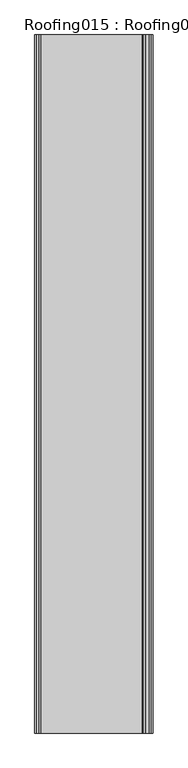
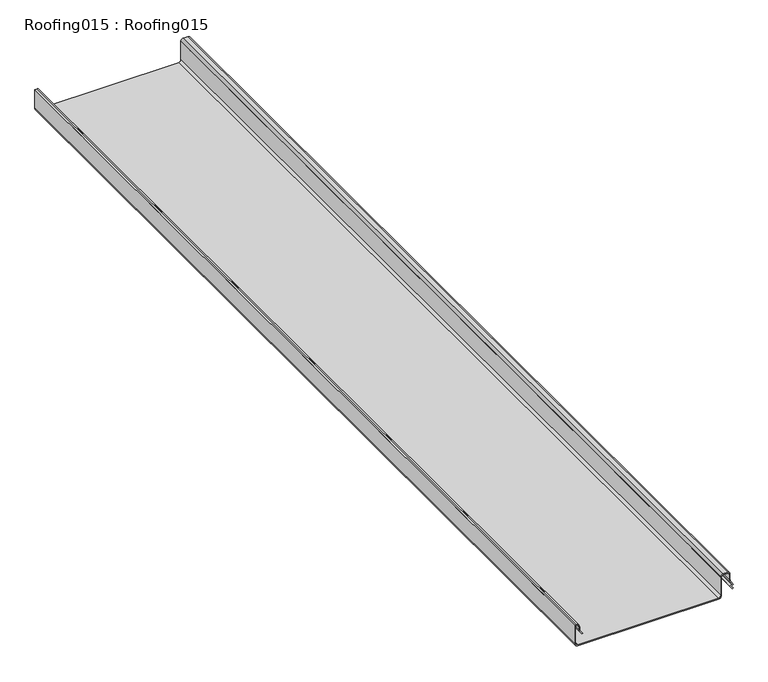
"""IFC4 building model written with IfcOpenShell, lengths in millimetres: proxy geometry, Roofing015 : Roofing015."""

from ifc_helpers import new_model, si_unit, point, frame, frame_2d, origin, place, context, project, spatial, polyline, circle_curve, trimmed, segment, composite_curve, outline, extrude, source, transform, mapped, element, save


def roofing015_roofing015_4853d511(model_context):
    return source(origin(), model_context, "Body", "SweptSolid", [
        extrude(outline(composite_curve([segment(polyline([(43493.0126404, 16767.0648158), (43484.5384782, 16773.2124644), (43485.7128993, 16774.8313329), (43494.1870614, 16768.6836843)]), True, "CONTINUOUS"), segment(trimmed(circle_curve(frame_2d((43495.9956699, 16771.1767417)), 3.08), [point((43494.1870614, 16768.6836843))], [point((43495.9956699, 16768.0967417))], True, "CARTESIAN"), True, "CONTINUOUS"), segment(polyline([(43495.9956699, 16768.0967417), (43502.7522282, 16768.0967417)]), True, "CONTINUOUS"), segment(trimmed(circle_curve(frame_2d((43502.7522282, 16761.0167417)), 7.08), [point((43502.7522282, 16768.0967417))], [point((43509.8322282, 16761.0167417))], False, "CARTESIAN"), True, "CONTINUOUS"), segment(polyline([(43509.8322282, 16761.0167417), (43509.8322282, 16757.421937), (43468.0950407, 16757.421937)]), True, "CONTINUOUS"), segment(trimmed(circle_curve(frame_2d((43468.0950407, 16764.501937)), 7.08), [point((43468.0950407, 16757.421937))], [point((43461.0150407, 16764.501937))], False, "CARTESIAN"), True, "CONTINUOUS"), segment(polyline([(43461.0150407, 16764.501937), (43461.0150407, 17064.7760191)]), True, "CONTINUOUS"), segment(trimmed(circle_curve(frame_2d((43468.0950407, 17064.7760191)), 7.08), [point((43461.0150407, 17064.7760191))], [point((43468.0950407, 17071.8560191))], False, "CARTESIAN"), True, "CONTINUOUS"), segment(polyline([(43468.0950407, 17071.8560191), (43509.7084782, 17071.8560191)]), True, "CONTINUOUS"), segment(trimmed(circle_curve(frame_2d((43509.7084782, 17074.9360191)), 3.08), [point((43509.7084782, 17071.8560191))], [point((43512.7884782, 17074.9360191))], True, "CARTESIAN"), True, "CONTINUOUS"), segment(polyline([(43512.7884782, 17074.9360191), (43512.7884782, 17084.943796)]), True, "CONTINUOUS"), segment(trimmed(circle_curve(frame_2d((43509.7084782, 17084.943796)), 3.08), [point((43512.7884782, 17084.943796))], [point((43509.7084782, 17088.023796))], True, "CARTESIAN"), True, "CONTINUOUS"), segment(polyline([(43509.7084782, 17088.023796), (43496.5259041, 17088.023796)]), True, "CONTINUOUS"), segment(trimmed(circle_curve(frame_2d((43496.5259041, 17095.103796)), 7.08), [point((43496.5259041, 17088.023796))], [point((43493.0360613, 17088.9436501))], False, "CARTESIAN"), True, "CONTINUOUS"), segment(polyline([(43493.0360613, 17088.9436501), (43484.1929304, 17093.9534561), (43481.6415322, 17089.6017913), (43474.259217, 17094.8721157), (43475.4212907, 17096.4998702), (43481.0228532, 17092.5008468), (43483.4642595, 17096.6649093), (43494.0218926, 17090.6838043)]), True, "CONTINUOUS"), segment(trimmed(circle_curve(frame_2d((43496.5259041, 17095.103796)), 5.08), [point((43494.0218926, 17090.6838043))], [point((43496.5259041, 17090.023796))], True, "CARTESIAN"), True, "CONTINUOUS"), segment(polyline([(43496.5259041, 17090.023796), (43509.7084782, 17090.023796)]), True, "CONTINUOUS"), segment(trimmed(circle_curve(frame_2d((43509.7084782, 17084.943796)), 5.08), [point((43509.7084782, 17090.023796))], [point((43514.7884782, 17084.943796))], False, "CARTESIAN"), True, "CONTINUOUS"), segment(polyline([(43514.7884782, 17084.943796), (43514.7884782, 17074.9360191)]), True, "CONTINUOUS"), segment(trimmed(circle_curve(frame_2d((43509.7084782, 17074.9360191)), 5.08), [point((43514.7884782, 17074.9360191))], [point((43509.7084782, 17069.8560191))], False, "CARTESIAN"), True, "CONTINUOUS"), segment(polyline([(43509.7084782, 17069.8560191), (43468.0950407, 17069.8560191)]), True, "CONTINUOUS"), segment(trimmed(circle_curve(frame_2d((43468.0950407, 17064.7760191)), 5.08), [point((43468.0950407, 17069.8560191))], [point((43463.0150407, 17064.7760191))], True, "CARTESIAN"), True, "CONTINUOUS"), segment(polyline([(43463.0150407, 17064.7760191), (43463.0150407, 16764.501937)]), True, "CONTINUOUS"), segment(trimmed(circle_curve(frame_2d((43468.0950407, 16764.501937)), 5.08), [point((43463.0150407, 16764.501937))], [point((43468.0950407, 16759.421937))], True, "CARTESIAN"), True, "CONTINUOUS"), segment(polyline([(43468.0950407, 16759.421937), (43507.8322282, 16759.421937), (43507.8322282, 16761.0167417)]), True, "CONTINUOUS"), segment(trimmed(circle_curve(frame_2d((43502.7522282, 16761.0167417)), 5.08), [point((43507.8322282, 16761.0167417))], [point((43502.7522282, 16766.0967417))], True, "CARTESIAN"), True, "CONTINUOUS"), segment(polyline([(43502.7522282, 16766.0967417), (43495.9956699, 16766.0967417)]), True, "CONTINUOUS"), segment(trimmed(circle_curve(frame_2d((43495.9956699, 16771.1767417)), 5.08), [point((43495.9956699, 16766.0967417))], [point((43493.0126404, 16767.0648158))], False, "CARTESIAN"), True, "CONTINUOUS")], self_intersect=False)), frame((0.0, 7982.1507711, 0.0), z_axis=(0.0, 1.0, 0.0), x_axis=(0.0, 0.0, 1.0)), (0.0, 0.0, 1.0), 2000.0),
    ])


if __name__ == "__main__":
    model = new_model("IFC4")
    model_context = context("Model", 3, world=origin())
    ifc_project = project(units=[si_unit("LENGTHUNIT", "METRE", prefix="MILLI")], contexts=[model_context])
    site = spatial("IfcSite", under=ifc_project)
    building = spatial("IfcBuilding", under=site)
    placement = place(None, origin())
    roofing015_roofing015_shape = roofing015_roofing015_4853d511(model_context)
    element("IfcBuildingElementProxy", 1, Name="Roofing015 : Roofing015", ObjectType="Roofing015 : Roofing015", at=placement, inside=building, context=model_context, shape_type="MappedRepresentation", body=[
        mapped(roofing015_roofing015_shape, transform((0.0, 0.0, 0.0), x_axis=(1.0, 0.0, 0.0), y_axis=(0.0, 1.0, 0.0), z_axis=(0.0, 0.0, 1.0))),
    ])
    save(model, "model.ifc")

# Revit data of these elements
# Type "Roofing015 : Roofing015"
#   NameOverride = "Roofing015"
# Element 1 (IfcBuildingElementProxy, "Roofing015 : Roofing015")
#   Materials on its faces: "STANDING SEAM METAL ROOF FOLLOW MANU. RECOMMENDED EDGE/TRANSITION DETAILS"
# Materials
#   "STANDING SEAM METAL ROOF FOLLOW MANU. RECOMMENDED EDGE/TRANSITION DETAILS": class "Unassigned", colour RGB 128 128 128, transparency 0, Cost = 0
